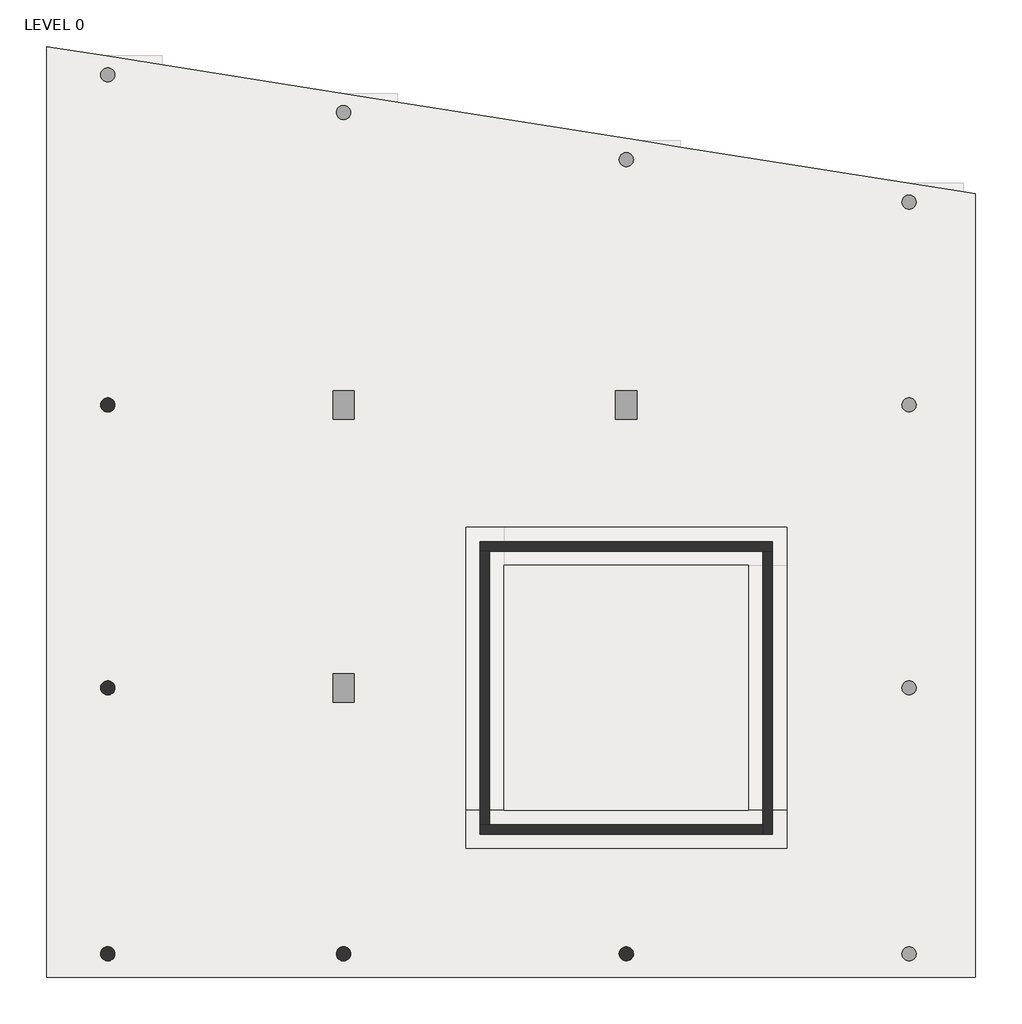
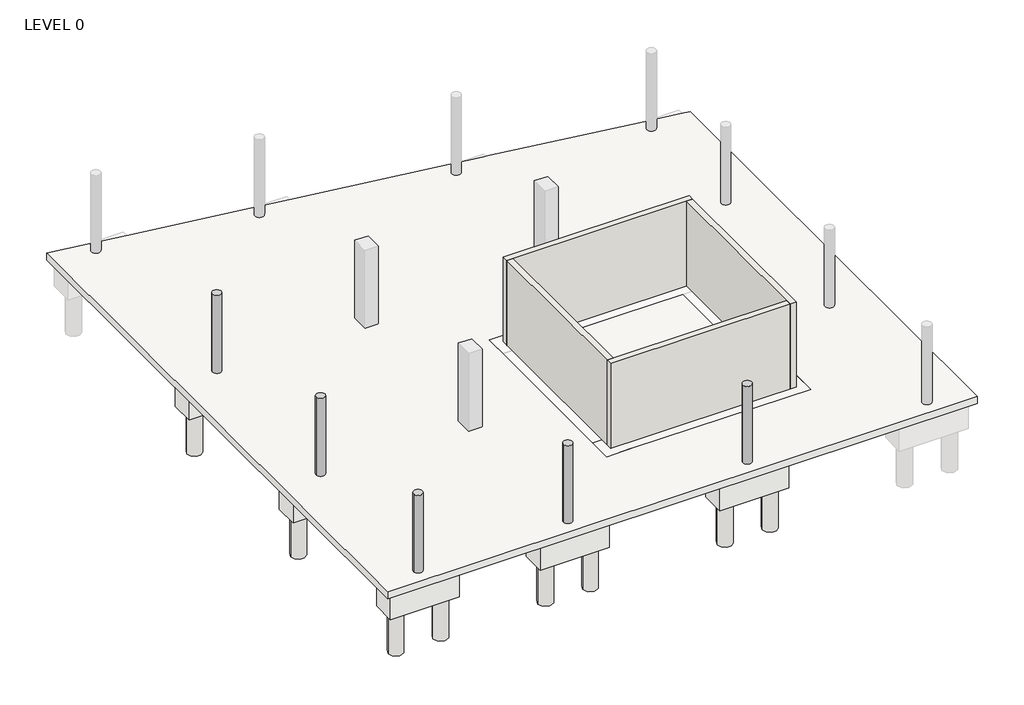
# One storey, part 1 of 3: 14 slabs, 5 columns, 4 walls, 1 footing.
"""IFC4 building model written with IfcOpenShell, lengths in millimetres."""

from ifc_helpers import new_model, si_unit, point, frame, frame_2d, origin, origin_with_axes, place, context, project, spatial, polyline, circle_curve, trimmed, segment, composite_curve, outline, extrude, faceted_brep, element, save
from ifc_brep_helpers import plane_surface, cylinder_surface, revolved_surface, advanced_brep

model = new_model("IFC4")

# Units and contexts
model_context = context("Model", 3, world=origin())
ifc_project = project(units=[si_unit("LENGTHUNIT", "METRE", prefix="MILLI")], contexts=[model_context])

# Site, building, storey
site = spatial("IfcSite", under=ifc_project)
building = spatial("IfcBuilding", under=site)
storey = spatial("IfcBuildingStorey", under=building, Name="LEVEL 0", Elevation=0.0)

# Columns
placement = place(None, origin())
element("IfcColumn", 1, ObjectType="BHm_StructuralColumns_ConcreteRound : 300 Ø RC COL", at=placement, inside=storey, context=model_context, shape_type="SweptSolid", body=[
    extrude(outline(composite_curve([segment(trimmed(circle_curve(frame_2d((-11075.1680269, 3000.0)), 150.0), [point((-11225.1680269, 3000.0))], [point((-10925.1680269, 3000.0))], False, "CARTESIAN"), True, "CONTINUOUS"), segment(trimmed(circle_curve(frame_2d((-11075.1680269, 3000.0)), 150.0), [point((-10925.1680269, 3000.0))], [point((-11225.1680269, 3000.0))], False, "CARTESIAN"), True, "CONTINUOUS")], self_intersect=False)), origin_with_axes(), (0.0, 0.0, 1.0), 2750.0),
])
element("IfcColumn", 2, ObjectType="BHm_StructuralColumns_ConcreteRound : 300 Ø RC COL", at=placement, inside=storey, context=model_context, shape_type="SweptSolid", body=[
    extrude(outline(composite_curve([segment(trimmed(circle_curve(frame_2d((-5075.1680269, 3000.0)), 150.0), [point((-5225.1680269, 3000.0))], [point((-4925.1680269, 3000.0))], False, "CARTESIAN"), True, "CONTINUOUS"), segment(trimmed(circle_curve(frame_2d((-5075.1680269, 3000.0)), 150.0), [point((-4925.1680269, 3000.0))], [point((-5225.1680269, 3000.0))], False, "CARTESIAN"), True, "CONTINUOUS")], self_intersect=False)), origin_with_axes(), (0.0, 0.0, 1.0), 2750.0),
])
element("IfcColumn", 3, ObjectType="BHm_StructuralColumns_ConcreteRound : 300 Ø RC COL", at=placement, inside=storey, context=model_context, shape_type="SweptSolid", body=[
    extrude(outline(composite_curve([segment(trimmed(circle_curve(frame_2d((-16075.1680269, 14640.7845261)), 150.0), [point((-16225.1680269, 14640.7845261))], [point((-15925.1680269, 14640.7845261))], False, "CARTESIAN"), True, "CONTINUOUS"), segment(trimmed(circle_curve(frame_2d((-16075.1680269, 14640.7845261)), 150.0), [point((-15925.1680269, 14640.7845261))], [point((-16225.1680269, 14640.7845261))], False, "CARTESIAN"), True, "CONTINUOUS")], self_intersect=False)), origin_with_axes(), (0.0, 0.0, 1.0), 2750.0),
])
element("IfcColumn", 4, ObjectType="BHm_StructuralColumns_ConcreteRound : 300 Ø RC COL", at=placement, inside=storey, context=model_context, shape_type="SweptSolid", body=[
    extrude(outline(composite_curve([segment(trimmed(circle_curve(frame_2d((-16075.1680269, 8640.7845261)), 150.0), [point((-16225.1680269, 8640.7845261))], [point((-15925.1680269, 8640.7845261))], False, "CARTESIAN"), True, "CONTINUOUS"), segment(trimmed(circle_curve(frame_2d((-16075.1680269, 8640.7845261)), 150.0), [point((-15925.1680269, 8640.7845261))], [point((-16225.1680269, 8640.7845261))], False, "CARTESIAN"), True, "CONTINUOUS")], self_intersect=False)), origin_with_axes(), (0.0, 0.0, 1.0), 2750.0),
])
element("IfcColumn", 5, ObjectType="BHm_StructuralColumns_ConcreteRound : 300 Ø RC COL", at=placement, inside=storey, context=model_context, shape_type="SweptSolid", body=[
    extrude(outline(composite_curve([segment(trimmed(circle_curve(frame_2d((-16075.1680269, 3000.0)), 150.0), [point((-16225.1680269, 3000.0))], [point((-15925.1680269, 3000.0))], False, "CARTESIAN"), True, "CONTINUOUS"), segment(trimmed(circle_curve(frame_2d((-16075.1680269, 3000.0)), 150.0), [point((-15925.1680269, 3000.0))], [point((-16225.1680269, 3000.0))], False, "CARTESIAN"), True, "CONTINUOUS")], self_intersect=False)), origin_with_axes(), (0.0, 0.0, 1.0), 2750.0),
])

# Footing
element("IfcFooting", 6, ObjectType="Wall Foundation", at=placement, inside=storey, context=model_context, shape_type="Brep", body=[
    faceted_brep([(-1670.3680269, 6045.5845261, 0.0), (-2479.9680269, 6045.5845261, 0.0), (-7670.3680269, 6045.5845261, 0.0), (-8479.9680269, 6045.5845261, 0.0), (-8479.9680269, 5235.9845261, 0.0), (-1670.3680269, 5235.9845261, 0.0), (-1670.3680269, 5235.9845261, -500.0), (-1670.3680269, 5235.9845261, -250.0), (-8479.9680269, 5235.9845261, -250.0), (-8479.9680269, 5235.9845261, -500.0), (-1670.3680269, 6045.5845261, -500.0), (-8479.9680269, 6045.5845261, -500.0)], [[[0, 1, 2, 3, 4, 5]], [[6, 7, 5, 4, 8, 9]], [[10, 6, 9, 11]], [[0, 10, 11, 3, 2, 1]], [[0, 5, 7, 6, 10]], [[4, 3, 11, 9, 8]]]),
])

# Slabs
element("IfcSlab", 7, ObjectType="BHm_StructuralFoundations_RC-2PileCap : 500Ø R.C. 2-PILE CAP", at=placement, inside=storey, context=model_context, shape_type="AdvancedBrep", body=[
    advanced_brep(
    [(-9925.1680269, 3400.0, -1100.0), (-9925.1680269, 2600.0, -1100.0), (-12225.1680269, 2600.0, -1100.0), (-12225.1680269, 3400.0, -1100.0), (-12075.1680269, 3000.0, -1100.0), (-11575.1680269, 3000.0, -1100.0), (-10575.1680269, 3000.0, -1100.0), (-10075.1680269, 3000.0, -1100.0), (-12225.1680269, 3400.0, -250.0), (-9925.1680269, 3400.0, -250.0), (-12225.1680269, 2600.0, -250.0), (-9925.1680269, 2600.0, -250.0), (-10575.1680269, 3000.0, -1025.0), (-10075.1680269, 3000.0, -1025.0), (-12075.1680269, 3000.0, -1025.0), (-11575.1680269, 3000.0, -1025.0)],
    [
        (0, 1),
        (1, 2),
        (2, 3),
        (3, 0),
        (4, 5, circle_curve(frame((-11825.1680269, 3000.0, -1100.0), z_axis=(0.0, 0.0, 1.0), x_axis=(1.0, 0.0, 0.0)), 250.0)),
        (5, 4, circle_curve(frame((-11825.1680269, 3000.0, -1100.0), z_axis=(0.0, 0.0, 1.0), x_axis=(1.0, 0.0, 0.0)), 250.0)),
        (6, 7, circle_curve(frame((-10325.1680269, 3000.0, -1100.0), z_axis=(0.0, 0.0, 1.0), x_axis=(1.0, 0.0, 0.0)), 250.0)),
        (7, 6, circle_curve(frame((-10325.1680269, 3000.0, -1100.0), z_axis=(0.0, 0.0, 1.0), x_axis=(1.0, 0.0, 0.0)), 250.0)),
        (3, 8),
        (8, 9),
        (9, 0),
        (2, 10),
        (10, 8),
        (1, 11),
        (11, 10),
        (9, 11),
        (12, 13, circle_curve(frame((-10325.1680269, 3000.0, -1025.0), z_axis=(0.0, 0.0, -1.0), x_axis=(1.0, 0.0, 0.0)), 250.0)),
        (13, 12, circle_curve(frame((-10325.1680269, 3000.0, -1025.0), z_axis=(0.0, 0.0, -1.0), x_axis=(1.0, 0.0, 0.0)), 250.0)),
        (4, 14),
        (14, 15, circle_curve(frame((-11825.1680269, 3000.0, -1025.0), z_axis=(0.0, 0.0, 1.0), x_axis=(1.0, 0.0, 0.0)), 250.0)),
        (15, 5),
        (15, 14, circle_curve(frame((-11825.1680269, 3000.0, -1025.0), z_axis=(0.0, 0.0, 1.0), x_axis=(1.0, 0.0, 0.0)), 250.0)),
        (6, 12),
        (13, 7),
    ],
    [
        plane_surface(frame((-12225.1680269, 3400.0, -1100.0), z_axis=(0.0, 0.0, -1.0), x_axis=(1.0, 0.0, 0.0))),
        plane_surface(frame((-9925.1680269, 3400.0, 0.0), z_axis=(0.0, 1.0, 0.0), x_axis=(0.0, 0.0, -1.0))),
        plane_surface(frame((-12225.1680269, 3400.0, 0.0), z_axis=(-1.0, 0.0, 0.0), x_axis=(0.0, 0.0, -1.0))),
        plane_surface(frame((-12225.1680269, 2600.0, 0.0), z_axis=(0.0, -1.0, 0.0), x_axis=(0.0, 0.0, -1.0))),
        plane_surface(frame((-9925.1680269, 2600.0, 0.0), z_axis=(1.0, 0.0, 0.0), x_axis=(0.0, 0.0, -1.0))),
        plane_surface(frame((-11575.1680269, 3000.0, -1025.0), z_axis=(0.0, 0.0, -1.0), x_axis=(0.0, 1.0, 0.0))),
        revolved_surface(polyline([(-11575.1680269, 3000.0, -1025.0), (-11575.1680269, 3000.0, -1100.0)]), (-11825.1680269, 3000.0, -1100.0), (0.0, 0.0, 1.0)),
        revolved_surface(polyline([(-10075.1680269, 3000.0, -1025.0), (-10075.1680269, 3000.0, -1100.0)]), (-10325.1680269, 3000.0, 0.0), (0.0, 0.0, 1.0)),
        plane_surface(frame((2324.8319731, 15140.7845261, -250.0), z_axis=(0.0, 0.0, 1.0), x_axis=(0.0, -1.0, 0.0))),
    ],
    [
        (0, [[1, 2, 3, 4], [5, 6], [7, 8]]),
        (1, [[-4, 9, 10, 11]]),
        (2, [[-3, 12, 13, -9]]),
        (3, [[-2, 14, 15, -12]]),
        (4, [[-1, -11, 16, -14]]),
        (5, [[17, 18]]),
        (6, [[-5, 19, 20, 21]]),
        (6, [[-6, -21, 22, -19]]),
        (7, [[-7, 23, -18, 24]]),
        (7, [[-8, -24, -17, -23]]),
        (8, [[-10, -13, -15, -16]]),
        (5, [[-22, -20]]),
    ],
),
])
element("IfcSlab", 8, ObjectType="BHm_StructuralFoundations_RC-Pile : 500Ø R.C. PILE", at=placement, inside=storey, context=model_context, shape_type="AdvancedBrep", body=[
    advanced_brep(
    [(-12075.1680269, 3000.0, -1025.0), (-11575.1680269, 3000.0, -1025.0), (-12075.1680269, 3000.0, -2600.0), (-11575.1680269, 3000.0, -2600.0), (-12075.1680269, 3000.0, -1100.0), (-11575.1680269, 3000.0, -1100.0)],
    [
        (0, 1, circle_curve(frame((-11825.1680269, 3000.0, -1025.0), z_axis=(0.0, 0.0, 1.0), x_axis=(1.0, 0.0, 0.0)), 250.0)),
        (1, 0, circle_curve(frame((-11825.1680269, 3000.0, -1025.0), z_axis=(0.0, 0.0, 1.0), x_axis=(1.0, 0.0, 0.0)), 250.0)),
        (2, 3, circle_curve(frame((-11825.1680269, 3000.0, -2600.0), z_axis=(0.0, 0.0, -1.0), x_axis=(1.0, 0.0, 0.0)), 250.0)),
        (3, 2, circle_curve(frame((-11825.1680269, 3000.0, -2600.0), z_axis=(0.0, 0.0, -1.0), x_axis=(1.0, 0.0, 0.0)), 250.0)),
        (0, 4),
        (4, 2),
        (3, 5),
        (5, 1),
    ],
    [
        plane_surface(frame((-11575.1680269, 3000.0, -1025.0), z_axis=(0.0, 0.0, 1.0), x_axis=(0.0, 1.0, 0.0))),
        plane_surface(frame((-11575.1680269, 3000.0, -2600.0), z_axis=(0.0, 0.0, -1.0), x_axis=(0.0, -1.0, 0.0))),
        cylinder_surface(frame((-11825.1680269, 3000.0, -2600.0), z_axis=(0.0, 0.0, 1.0), x_axis=(1.0, 0.0, 0.0)), 250.0),
    ],
    [
        (0, [[1, 2]]),
        (1, [[3, 4]]),
        (2, [[-1, 5, 6, -4, 7, 8]]),
        (2, [[-2, -8, -7, -3, -6, -5]]),
    ],
),
])
element("IfcSlab", 9, ObjectType="BHm_StructuralFoundations_RC-Pile : 500Ø R.C. PILE", at=placement, inside=storey, context=model_context, shape_type="AdvancedBrep", body=[
    advanced_brep(
    [(-10575.1680269, 3000.0, -1025.0), (-10075.1680269, 3000.0, -1025.0), (-10575.1680269, 3000.0, -2600.0), (-10075.1680269, 3000.0, -2600.0), (-10575.1680269, 3000.0, -1100.0), (-10075.1680269, 3000.0, -1100.0)],
    [
        (0, 1, circle_curve(frame((-10325.1680269, 3000.0, -1025.0), z_axis=(0.0, 0.0, 1.0), x_axis=(1.0, 0.0, 0.0)), 250.0)),
        (1, 0, circle_curve(frame((-10325.1680269, 3000.0, -1025.0), z_axis=(0.0, 0.0, 1.0), x_axis=(1.0, 0.0, 0.0)), 250.0)),
        (2, 3, circle_curve(frame((-10325.1680269, 3000.0, -2600.0), z_axis=(0.0, 0.0, -1.0), x_axis=(1.0, 0.0, 0.0)), 250.0)),
        (3, 2, circle_curve(frame((-10325.1680269, 3000.0, -2600.0), z_axis=(0.0, 0.0, -1.0), x_axis=(1.0, 0.0, 0.0)), 250.0)),
        (0, 4),
        (4, 2),
        (3, 5),
        (5, 1),
    ],
    [
        plane_surface(frame((-10075.1680269, 3000.0, -1025.0), z_axis=(0.0, 0.0, 1.0), x_axis=(0.0, 1.0, 0.0))),
        plane_surface(frame((-10075.1680269, 3000.0, -2600.0), z_axis=(0.0, 0.0, -1.0), x_axis=(0.0, -1.0, 0.0))),
        cylinder_surface(frame((-10325.1680269, 3000.0, -2600.0), z_axis=(0.0, 0.0, 1.0), x_axis=(1.0, 0.0, 0.0)), 250.0),
    ],
    [
        (0, [[1, 2]]),
        (1, [[3, 4]]),
        (2, [[-1, 5, 6, -4, 7, 8]]),
        (2, [[-2, -8, -7, -3, -6, -5]]),
    ],
),
])
element("IfcSlab", 10, ObjectType="BHm_StructuralFoundations_RC-2PileCap : 500Ø R.C. 2-PILE CAP", at=placement, inside=storey, context=model_context, shape_type="AdvancedBrep", body=[
    advanced_brep(
    [(-3925.1680269, 3400.0, -1100.0), (-3925.1680269, 2600.0, -1100.0), (-6225.1680269, 2600.0, -1100.0), (-6225.1680269, 3400.0, -1100.0), (-6075.1680269, 3000.0, -1100.0), (-5575.1680269, 3000.0, -1100.0), (-4575.1680269, 3000.0, -1100.0), (-4075.1680269, 3000.0, -1100.0), (-6225.1680269, 3400.0, -250.0), (-3925.1680269, 3400.0, -250.0), (-6225.1680269, 2600.0, -250.0), (-3925.1680269, 2600.0, -250.0), (-4575.1680269, 3000.0, -1025.0), (-4075.1680269, 3000.0, -1025.0), (-6075.1680269, 3000.0, -1025.0), (-5575.1680269, 3000.0, -1025.0)],
    [
        (0, 1),
        (1, 2),
        (2, 3),
        (3, 0),
        (4, 5, circle_curve(frame((-5825.1680269, 3000.0, -1100.0), z_axis=(0.0, 0.0, 1.0), x_axis=(1.0, 0.0, 0.0)), 250.0)),
        (5, 4, circle_curve(frame((-5825.1680269, 3000.0, -1100.0), z_axis=(0.0, 0.0, 1.0), x_axis=(1.0, 0.0, 0.0)), 250.0)),
        (6, 7, circle_curve(frame((-4325.1680269, 3000.0, -1100.0), z_axis=(0.0, 0.0, 1.0), x_axis=(1.0, 0.0, 0.0)), 250.0)),
        (7, 6, circle_curve(frame((-4325.1680269, 3000.0, -1100.0), z_axis=(0.0, 0.0, 1.0), x_axis=(1.0, 0.0, 0.0)), 250.0)),
        (3, 8),
        (8, 9),
        (9, 0),
        (2, 10),
        (10, 8),
        (1, 11),
        (11, 10),
        (9, 11),
        (12, 13, circle_curve(frame((-4325.1680269, 3000.0, -1025.0), z_axis=(0.0, 0.0, -1.0), x_axis=(1.0, 0.0, 0.0)), 250.0)),
        (13, 12, circle_curve(frame((-4325.1680269, 3000.0, -1025.0), z_axis=(0.0, 0.0, -1.0), x_axis=(1.0, 0.0, 0.0)), 250.0)),
        (4, 14),
        (14, 15, circle_curve(frame((-5825.1680269, 3000.0, -1025.0), z_axis=(0.0, 0.0, 1.0), x_axis=(1.0, 0.0, 0.0)), 250.0)),
        (15, 5),
        (15, 14, circle_curve(frame((-5825.1680269, 3000.0, -1025.0), z_axis=(0.0, 0.0, 1.0), x_axis=(1.0, 0.0, 0.0)), 250.0)),
        (6, 12),
        (13, 7),
    ],
    [
        plane_surface(frame((-6225.1680269, 3400.0, -1100.0), z_axis=(0.0, 0.0, -1.0), x_axis=(1.0, 0.0, 0.0))),
        plane_surface(frame((-3925.1680269, 3400.0, 0.0), z_axis=(0.0, 1.0, 0.0), x_axis=(0.0, 0.0, -1.0))),
        plane_surface(frame((-6225.1680269, 3400.0, 0.0), z_axis=(-1.0, 0.0, 0.0), x_axis=(0.0, 0.0, -1.0))),
        plane_surface(frame((-6225.1680269, 2600.0, 0.0), z_axis=(0.0, -1.0, 0.0), x_axis=(0.0, 0.0, -1.0))),
        plane_surface(frame((-3925.1680269, 2600.0, 0.0), z_axis=(1.0, 0.0, 0.0), x_axis=(0.0, 0.0, -1.0))),
        plane_surface(frame((-5575.1680269, 3000.0, -1025.0), z_axis=(0.0, 0.0, -1.0), x_axis=(0.0, 1.0, 0.0))),
        revolved_surface(polyline([(-5575.1680269, 3000.0, -1025.0), (-5575.1680269, 3000.0, -1100.0)]), (-5825.1680269, 3000.0, -1100.0), (0.0, 0.0, 1.0)),
        revolved_surface(polyline([(-4075.1680269, 3000.0, -1025.0), (-4075.1680269, 3000.0, -1100.0)]), (-4325.1680269, 3000.0, 0.0), (0.0, 0.0, 1.0)),
        plane_surface(frame((2324.8319731, 15140.7845261, -250.0), z_axis=(0.0, 0.0, 1.0), x_axis=(0.0, -1.0, 0.0))),
    ],
    [
        (0, [[1, 2, 3, 4], [5, 6], [7, 8]]),
        (1, [[-4, 9, 10, 11]]),
        (2, [[-3, 12, 13, -9]]),
        (3, [[-2, 14, 15, -12]]),
        (4, [[-1, -11, 16, -14]]),
        (5, [[17, 18]]),
        (6, [[-5, 19, 20, 21]]),
        (6, [[-6, -21, 22, -19]]),
        (7, [[-7, 23, -18, 24]]),
        (7, [[-8, -24, -17, -23]]),
        (8, [[-10, -13, -15, -16]]),
        (5, [[-22, -20]]),
    ],
),
])
element("IfcSlab", 11, ObjectType="BHm_StructuralFoundations_RC-Pile : 500Ø R.C. PILE", at=placement, inside=storey, context=model_context, shape_type="AdvancedBrep", body=[
    advanced_brep(
    [(-6075.1680269, 3000.0, -1025.0), (-5575.1680269, 3000.0, -1025.0), (-6075.1680269, 3000.0, -2600.0), (-5575.1680269, 3000.0, -2600.0), (-6075.1680269, 3000.0, -1100.0), (-5575.1680269, 3000.0, -1100.0)],
    [
        (0, 1, circle_curve(frame((-5825.1680269, 3000.0, -1025.0), z_axis=(0.0, 0.0, 1.0), x_axis=(1.0, 0.0, 0.0)), 250.0)),
        (1, 0, circle_curve(frame((-5825.1680269, 3000.0, -1025.0), z_axis=(0.0, 0.0, 1.0), x_axis=(1.0, 0.0, 0.0)), 250.0)),
        (2, 3, circle_curve(frame((-5825.1680269, 3000.0, -2600.0), z_axis=(0.0, 0.0, -1.0), x_axis=(1.0, 0.0, 0.0)), 250.0)),
        (3, 2, circle_curve(frame((-5825.1680269, 3000.0, -2600.0), z_axis=(0.0, 0.0, -1.0), x_axis=(1.0, 0.0, 0.0)), 250.0)),
        (0, 4),
        (4, 2),
        (3, 5),
        (5, 1),
    ],
    [
        plane_surface(frame((-5575.1680269, 3000.0, -1025.0), z_axis=(0.0, 0.0, 1.0), x_axis=(0.0, 1.0, 0.0))),
        plane_surface(frame((-5575.1680269, 3000.0, -2600.0), z_axis=(0.0, 0.0, -1.0), x_axis=(0.0, -1.0, 0.0))),
        cylinder_surface(frame((-5825.1680269, 3000.0, -2600.0), z_axis=(0.0, 0.0, 1.0), x_axis=(1.0, 0.0, 0.0)), 250.0),
    ],
    [
        (0, [[1, 2]]),
        (1, [[3, 4]]),
        (2, [[-1, 5, 6, -4, 7, 8]]),
        (2, [[-2, -8, -7, -3, -6, -5]]),
    ],
),
])
element("IfcSlab", 12, ObjectType="BHm_StructuralFoundations_RC-Pile : 500Ø R.C. PILE", at=placement, inside=storey, context=model_context, shape_type="AdvancedBrep", body=[
    advanced_brep(
    [(-4575.1680269, 3000.0, -1025.0), (-4075.1680269, 3000.0, -1025.0), (-4575.1680269, 3000.0, -2600.0), (-4075.1680269, 3000.0, -2600.0), (-4575.1680269, 3000.0, -1100.0), (-4075.1680269, 3000.0, -1100.0)],
    [
        (0, 1, circle_curve(frame((-4325.1680269, 3000.0, -1025.0), z_axis=(0.0, 0.0, 1.0), x_axis=(1.0, 0.0, 0.0)), 250.0)),
        (1, 0, circle_curve(frame((-4325.1680269, 3000.0, -1025.0), z_axis=(0.0, 0.0, 1.0), x_axis=(1.0, 0.0, 0.0)), 250.0)),
        (2, 3, circle_curve(frame((-4325.1680269, 3000.0, -2600.0), z_axis=(0.0, 0.0, -1.0), x_axis=(1.0, 0.0, 0.0)), 250.0)),
        (3, 2, circle_curve(frame((-4325.1680269, 3000.0, -2600.0), z_axis=(0.0, 0.0, -1.0), x_axis=(1.0, 0.0, 0.0)), 250.0)),
        (0, 4),
        (4, 2),
        (3, 5),
        (5, 1),
    ],
    [
        plane_surface(frame((-4075.1680269, 3000.0, -1025.0), z_axis=(0.0, 0.0, 1.0), x_axis=(0.0, 1.0, 0.0))),
        plane_surface(frame((-4075.1680269, 3000.0, -2600.0), z_axis=(0.0, 0.0, -1.0), x_axis=(0.0, -1.0, 0.0))),
        cylinder_surface(frame((-4325.1680269, 3000.0, -2600.0), z_axis=(0.0, 0.0, 1.0), x_axis=(1.0, 0.0, 0.0)), 250.0),
    ],
    [
        (0, [[1, 2]]),
        (1, [[3, 4]]),
        (2, [[-1, 5, 6, -4, 7, 8]]),
        (2, [[-2, -8, -7, -3, -6, -5]]),
    ],
),
])
element("IfcSlab", 13, ObjectType="BHm_StructuralFoundations_RC-2PileCap : 500Ø R.C. 2-PILE CAP", at=placement, inside=storey, context=model_context, shape_type="AdvancedBrep", body=[
    advanced_brep(
    [(-14925.1680269, 15040.7845261, -1100.0), (-14925.1680269, 14240.7845261, -1100.0), (-17225.1680269, 14240.7845261, -1100.0), (-17225.1680269, 15040.7845261, -1100.0), (-17075.1680269, 14640.7845261, -1100.0), (-16575.1680269, 14640.7845261, -1100.0), (-15575.1680269, 14640.7845261, -1100.0), (-15075.1680269, 14640.7845261, -1100.0), (-17225.1680269, 15040.7845261, -250.0), (-14925.1680269, 15040.7845261, -250.0), (-17225.1680269, 14240.7845261, -250.0), (-14925.1680269, 14240.7845261, -250.0), (-15575.1680269, 14640.7845261, -1025.0), (-15075.1680269, 14640.7845261, -1025.0), (-17075.1680269, 14640.7845261, -1025.0), (-16575.1680269, 14640.7845261, -1025.0)],
    [
        (0, 1),
        (1, 2),
        (2, 3),
        (3, 0),
        (4, 5, circle_curve(frame((-16825.1680269, 14640.7845261, -1100.0), z_axis=(0.0, 0.0, 1.0), x_axis=(1.0, 0.0, 0.0)), 250.0)),
        (5, 4, circle_curve(frame((-16825.1680269, 14640.7845261, -1100.0), z_axis=(0.0, 0.0, 1.0), x_axis=(1.0, 0.0, 0.0)), 250.0)),
        (6, 7, circle_curve(frame((-15325.1680269, 14640.7845261, -1100.0), z_axis=(0.0, 0.0, 1.0), x_axis=(1.0, 0.0, 0.0)), 250.0)),
        (7, 6, circle_curve(frame((-15325.1680269, 14640.7845261, -1100.0), z_axis=(0.0, 0.0, 1.0), x_axis=(1.0, 0.0, 0.0)), 250.0)),
        (3, 8),
        (8, 9),
        (9, 0),
        (2, 10),
        (10, 8),
        (1, 11),
        (11, 10),
        (9, 11),
        (12, 13, circle_curve(frame((-15325.1680269, 14640.7845261, -1025.0), z_axis=(0.0, 0.0, -1.0), x_axis=(1.0, 0.0, 0.0)), 250.0)),
        (13, 12, circle_curve(frame((-15325.1680269, 14640.7845261, -1025.0), z_axis=(0.0, 0.0, -1.0), x_axis=(1.0, 0.0, 0.0)), 250.0)),
        (4, 14),
        (14, 15, circle_curve(frame((-16825.1680269, 14640.7845261, -1025.0), z_axis=(0.0, 0.0, 1.0), x_axis=(1.0, 0.0, 0.0)), 250.0)),
        (15, 5),
        (15, 14, circle_curve(frame((-16825.1680269, 14640.7845261, -1025.0), z_axis=(0.0, 0.0, 1.0), x_axis=(1.0, 0.0, 0.0)), 250.0)),
        (6, 12),
        (13, 7),
    ],
    [
        plane_surface(frame((-17225.1680269, 15040.7845261, -1100.0), z_axis=(0.0, 0.0, -1.0), x_axis=(1.0, 0.0, 0.0))),
        plane_surface(frame((-14925.1680269, 15040.7845261, 0.0), z_axis=(0.0, 1.0, 0.0), x_axis=(0.0, 0.0, -1.0))),
        plane_surface(frame((-17225.1680269, 15040.7845261, 0.0), z_axis=(-1.0, 0.0, 0.0), x_axis=(0.0, 0.0, -1.0))),
        plane_surface(frame((-17225.1680269, 14240.7845261, 0.0), z_axis=(0.0, -1.0, 0.0), x_axis=(0.0, 0.0, -1.0))),
        plane_surface(frame((-14925.1680269, 14240.7845261, 0.0), z_axis=(1.0, 0.0, 0.0), x_axis=(0.0, 0.0, -1.0))),
        plane_surface(frame((-16575.1680269, 14640.7845261, -1025.0), z_axis=(0.0, 0.0, -1.0), x_axis=(0.0, 1.0, 0.0))),
        revolved_surface(polyline([(-16575.1680269, 14640.7845261, -1025.0), (-16575.1680269, 14640.7845261, -1100.0)]), (-16825.1680269, 14640.7845261, -1100.0), (0.0, 0.0, 1.0)),
        revolved_surface(polyline([(-15075.1680269, 14640.7845261, -1025.0), (-15075.1680269, 14640.7845261, -1100.0)]), (-15325.1680269, 14640.7845261, 0.0), (0.0, 0.0, 1.0)),
        plane_surface(frame((2324.8319731, 15140.7845261, -250.0), z_axis=(0.0, 0.0, 1.0), x_axis=(0.0, -1.0, 0.0))),
    ],
    [
        (0, [[1, 2, 3, 4], [5, 6], [7, 8]]),
        (1, [[-4, 9, 10, 11]]),
        (2, [[-3, 12, 13, -9]]),
        (3, [[-2, 14, 15, -12]]),
        (4, [[-1, -11, 16, -14]]),
        (5, [[17, 18]]),
        (6, [[-5, 19, 20, 21]]),
        (6, [[-6, -21, 22, -19]]),
        (7, [[-7, 23, -18, 24]]),
        (7, [[-8, -24, -17, -23]]),
        (8, [[-10, -13, -15, -16]]),
        (5, [[-22, -20]]),
    ],
),
])
element("IfcSlab", 14, ObjectType="BHm_StructuralFoundations_RC-Pile : 500Ø R.C. PILE", at=placement, inside=storey, context=model_context, shape_type="AdvancedBrep", body=[
    advanced_brep(
    [(-17075.1680269, 14640.7845261, -1025.0), (-16575.1680269, 14640.7845261, -1025.0), (-17075.1680269, 14640.7845261, -2600.0), (-16575.1680269, 14640.7845261, -2600.0), (-17075.1680269, 14640.7845261, -1100.0), (-16575.1680269, 14640.7845261, -1100.0)],
    [
        (0, 1, circle_curve(frame((-16825.1680269, 14640.7845261, -1025.0), z_axis=(0.0, 0.0, 1.0), x_axis=(1.0, 0.0, 0.0)), 250.0)),
        (1, 0, circle_curve(frame((-16825.1680269, 14640.7845261, -1025.0), z_axis=(0.0, 0.0, 1.0), x_axis=(1.0, 0.0, 0.0)), 250.0)),
        (2, 3, circle_curve(frame((-16825.1680269, 14640.7845261, -2600.0), z_axis=(0.0, 0.0, -1.0), x_axis=(1.0, 0.0, 0.0)), 250.0)),
        (3, 2, circle_curve(frame((-16825.1680269, 14640.7845261, -2600.0), z_axis=(0.0, 0.0, -1.0), x_axis=(1.0, 0.0, 0.0)), 250.0)),
        (0, 4),
        (4, 2),
        (3, 5),
        (5, 1),
    ],
    [
        plane_surface(frame((-16575.1680269, 14640.7845261, -1025.0), z_axis=(0.0, 0.0, 1.0), x_axis=(0.0, 1.0, 0.0))),
        plane_surface(frame((-16575.1680269, 14640.7845261, -2600.0), z_axis=(0.0, 0.0, -1.0), x_axis=(0.0, -1.0, 0.0))),
        cylinder_surface(frame((-16825.1680269, 14640.7845261, -2600.0), z_axis=(0.0, 0.0, 1.0), x_axis=(1.0, 0.0, 0.0)), 250.0),
    ],
    [
        (0, [[1, 2]]),
        (1, [[3, 4]]),
        (2, [[-1, 5, 6, -4, 7, 8]]),
        (2, [[-2, -8, -7, -3, -6, -5]]),
    ],
),
])
element("IfcSlab", 15, ObjectType="BHm_StructuralFoundations_RC-2PileCap : 500Ø R.C. 2-PILE CAP", at=placement, inside=storey, context=model_context, shape_type="AdvancedBrep", body=[
    advanced_brep(
    [(-14925.1680269, 9040.7845261, -1100.0), (-14925.1680269, 8240.7845261, -1100.0), (-17225.1680269, 8240.7845261, -1100.0), (-17225.1680269, 9040.7845261, -1100.0), (-17075.1680269, 8640.7845261, -1100.0), (-16575.1680269, 8640.7845261, -1100.0), (-15575.1680269, 8640.7845261, -1100.0), (-15075.1680269, 8640.7845261, -1100.0), (-17225.1680269, 9040.7845261, -250.0), (-14925.1680269, 9040.7845261, -250.0), (-17225.1680269, 8240.7845261, -250.0), (-14925.1680269, 8240.7845261, -250.0), (-15575.1680269, 8640.7845261, -1025.0), (-15075.1680269, 8640.7845261, -1025.0), (-17075.1680269, 8640.7845261, -1025.0), (-16575.1680269, 8640.7845261, -1025.0)],
    [
        (0, 1),
        (1, 2),
        (2, 3),
        (3, 0),
        (4, 5, circle_curve(frame((-16825.1680269, 8640.7845261, -1100.0), z_axis=(0.0, 0.0, 1.0), x_axis=(1.0, 0.0, 0.0)), 250.0)),
        (5, 4, circle_curve(frame((-16825.1680269, 8640.7845261, -1100.0), z_axis=(0.0, 0.0, 1.0), x_axis=(1.0, 0.0, 0.0)), 250.0)),
        (6, 7, circle_curve(frame((-15325.1680269, 8640.7845261, -1100.0), z_axis=(0.0, 0.0, 1.0), x_axis=(1.0, 0.0, 0.0)), 250.0)),
        (7, 6, circle_curve(frame((-15325.1680269, 8640.7845261, -1100.0), z_axis=(0.0, 0.0, 1.0), x_axis=(1.0, 0.0, 0.0)), 250.0)),
        (3, 8),
        (8, 9),
        (9, 0),
        (2, 10),
        (10, 8),
        (1, 11),
        (11, 10),
        (9, 11),
        (12, 13, circle_curve(frame((-15325.1680269, 8640.7845261, -1025.0), z_axis=(0.0, 0.0, -1.0), x_axis=(1.0, 0.0, 0.0)), 250.0)),
        (13, 12, circle_curve(frame((-15325.1680269, 8640.7845261, -1025.0), z_axis=(0.0, 0.0, -1.0), x_axis=(1.0, 0.0, 0.0)), 250.0)),
        (4, 14),
        (14, 15, circle_curve(frame((-16825.1680269, 8640.7845261, -1025.0), z_axis=(0.0, 0.0, 1.0), x_axis=(1.0, 0.0, 0.0)), 250.0)),
        (15, 5),
        (15, 14, circle_curve(frame((-16825.1680269, 8640.7845261, -1025.0), z_axis=(0.0, 0.0, 1.0), x_axis=(1.0, 0.0, 0.0)), 250.0)),
        (6, 12),
        (13, 7),
    ],
    [
        plane_surface(frame((-17225.1680269, 9040.7845261, -1100.0), z_axis=(0.0, 0.0, -1.0), x_axis=(1.0, 0.0, 0.0))),
        plane_surface(frame((-14925.1680269, 9040.7845261, 0.0), z_axis=(0.0, 1.0, 0.0), x_axis=(0.0, 0.0, -1.0))),
        plane_surface(frame((-17225.1680269, 9040.7845261, 0.0), z_axis=(-1.0, 0.0, 0.0), x_axis=(0.0, 0.0, -1.0))),
        plane_surface(frame((-17225.1680269, 8240.7845261, 0.0), z_axis=(0.0, -1.0, 0.0), x_axis=(0.0, 0.0, -1.0))),
        plane_surface(frame((-14925.1680269, 8240.7845261, 0.0), z_axis=(1.0, 0.0, 0.0), x_axis=(0.0, 0.0, -1.0))),
        plane_surface(frame((-16575.1680269, 8640.7845261, -1025.0), z_axis=(0.0, 0.0, -1.0), x_axis=(0.0, 1.0, 0.0))),
        revolved_surface(polyline([(-16575.1680269, 8640.7845261, -1025.0), (-16575.1680269, 8640.7845261, -1100.0)]), (-16825.1680269, 8640.7845261, -1100.0), (0.0, 0.0, 1.0)),
        revolved_surface(polyline([(-15075.1680269, 8640.7845261, -1025.0), (-15075.1680269, 8640.7845261, -1100.0)]), (-15325.1680269, 8640.7845261, 0.0), (0.0, 0.0, 1.0)),
        plane_surface(frame((2324.8319731, 15140.7845261, -250.0), z_axis=(0.0, 0.0, 1.0), x_axis=(0.0, -1.0, 0.0))),
    ],
    [
        (0, [[1, 2, 3, 4], [5, 6], [7, 8]]),
        (1, [[-4, 9, 10, 11]]),
        (2, [[-3, 12, 13, -9]]),
        (3, [[-2, 14, 15, -12]]),
        (4, [[-1, -11, 16, -14]]),
        (5, [[17, 18]]),
        (6, [[-5, 19, 20, 21]]),
        (6, [[-6, -21, 22, -19]]),
        (7, [[-7, 23, -18, 24]]),
        (7, [[-8, -24, -17, -23]]),
        (8, [[-10, -13, -15, -16]]),
        (5, [[-22, -20]]),
    ],
),
])
element("IfcSlab", 16, ObjectType="BHm_StructuralFoundations_RC-Pile : 500Ø R.C. PILE", at=placement, inside=storey, context=model_context, shape_type="AdvancedBrep", body=[
    advanced_brep(
    [(-17075.1680269, 8640.7845261, -1025.0), (-16575.1680269, 8640.7845261, -1025.0), (-17075.1680269, 8640.7845261, -2600.0), (-16575.1680269, 8640.7845261, -2600.0), (-17075.1680269, 8640.7845261, -1100.0), (-16575.1680269, 8640.7845261, -1100.0)],
    [
        (0, 1, circle_curve(frame((-16825.1680269, 8640.7845261, -1025.0), z_axis=(0.0, 0.0, 1.0), x_axis=(1.0, 0.0, 0.0)), 250.0)),
        (1, 0, circle_curve(frame((-16825.1680269, 8640.7845261, -1025.0), z_axis=(0.0, 0.0, 1.0), x_axis=(1.0, 0.0, 0.0)), 250.0)),
        (2, 3, circle_curve(frame((-16825.1680269, 8640.7845261, -2600.0), z_axis=(0.0, 0.0, -1.0), x_axis=(1.0, 0.0, 0.0)), 250.0)),
        (3, 2, circle_curve(frame((-16825.1680269, 8640.7845261, -2600.0), z_axis=(0.0, 0.0, -1.0), x_axis=(1.0, 0.0, 0.0)), 250.0)),
        (0, 4),
        (4, 2),
        (3, 5),
        (5, 1),
    ],
    [
        plane_surface(frame((-16575.1680269, 8640.7845261, -1025.0), z_axis=(0.0, 0.0, 1.0), x_axis=(0.0, 1.0, 0.0))),
        plane_surface(frame((-16575.1680269, 8640.7845261, -2600.0), z_axis=(0.0, 0.0, -1.0), x_axis=(0.0, -1.0, 0.0))),
        cylinder_surface(frame((-16825.1680269, 8640.7845261, -2600.0), z_axis=(0.0, 0.0, 1.0), x_axis=(1.0, 0.0, 0.0)), 250.0),
    ],
    [
        (0, [[1, 2]]),
        (1, [[3, 4]]),
        (2, [[-1, 5, 6, -4, 7, 8]]),
        (2, [[-2, -8, -7, -3, -6, -5]]),
    ],
),
])
element("IfcSlab", 17, ObjectType="BHm_StructuralFoundations_RC-2PileCap : 500Ø R.C. 2-PILE CAP", at=placement, inside=storey, context=model_context, shape_type="AdvancedBrep", body=[
    advanced_brep(
    [(-14925.1680269, 3400.0, -1100.0), (-14925.1680269, 2600.0, -1100.0), (-17225.1680269, 2600.0, -1100.0), (-17225.1680269, 3400.0, -1100.0), (-17075.1680269, 3000.0, -1100.0), (-16575.1680269, 3000.0, -1100.0), (-15575.1680269, 3000.0, -1100.0), (-15075.1680269, 3000.0, -1100.0), (-17225.1680269, 3400.0, -250.0), (-14925.1680269, 3400.0, -250.0), (-17225.1680269, 2600.0, -250.0), (-14925.1680269, 2600.0, -250.0), (-15575.1680269, 3000.0, -1025.0), (-15075.1680269, 3000.0, -1025.0), (-17075.1680269, 3000.0, -1025.0), (-16575.1680269, 3000.0, -1025.0)],
    [
        (0, 1),
        (1, 2),
        (2, 3),
        (3, 0),
        (4, 5, circle_curve(frame((-16825.1680269, 3000.0, -1100.0), z_axis=(0.0, 0.0, 1.0), x_axis=(1.0, 0.0, 0.0)), 250.0)),
        (5, 4, circle_curve(frame((-16825.1680269, 3000.0, -1100.0), z_axis=(0.0, 0.0, 1.0), x_axis=(1.0, 0.0, 0.0)), 250.0)),
        (6, 7, circle_curve(frame((-15325.1680269, 3000.0, -1100.0), z_axis=(0.0, 0.0, 1.0), x_axis=(1.0, 0.0, 0.0)), 250.0)),
        (7, 6, circle_curve(frame((-15325.1680269, 3000.0, -1100.0), z_axis=(0.0, 0.0, 1.0), x_axis=(1.0, 0.0, 0.0)), 250.0)),
        (3, 8),
        (8, 9),
        (9, 0),
        (2, 10),
        (10, 8),
        (1, 11),
        (11, 10),
        (9, 11),
        (12, 13, circle_curve(frame((-15325.1680269, 3000.0, -1025.0), z_axis=(0.0, 0.0, -1.0), x_axis=(1.0, 0.0, 0.0)), 250.0)),
        (13, 12, circle_curve(frame((-15325.1680269, 3000.0, -1025.0), z_axis=(0.0, 0.0, -1.0), x_axis=(1.0, 0.0, 0.0)), 250.0)),
        (4, 14),
        (14, 15, circle_curve(frame((-16825.1680269, 3000.0, -1025.0), z_axis=(0.0, 0.0, 1.0), x_axis=(1.0, 0.0, 0.0)), 250.0)),
        (15, 5),
        (15, 14, circle_curve(frame((-16825.1680269, 3000.0, -1025.0), z_axis=(0.0, 0.0, 1.0), x_axis=(1.0, 0.0, 0.0)), 250.0)),
        (6, 12),
        (13, 7),
    ],
    [
        plane_surface(frame((-17225.1680269, 3400.0, -1100.0), z_axis=(0.0, 0.0, -1.0), x_axis=(1.0, 0.0, 0.0))),
        plane_surface(frame((-14925.1680269, 3400.0, 0.0), z_axis=(0.0, 1.0, 0.0), x_axis=(0.0, 0.0, -1.0))),
        plane_surface(frame((-17225.1680269, 3400.0, 0.0), z_axis=(-1.0, 0.0, 0.0), x_axis=(0.0, 0.0, -1.0))),
        plane_surface(frame((-17225.1680269, 2600.0, 0.0), z_axis=(0.0, -1.0, 0.0), x_axis=(0.0, 0.0, -1.0))),
        plane_surface(frame((-14925.1680269, 2600.0, 0.0), z_axis=(1.0, 0.0, 0.0), x_axis=(0.0, 0.0, -1.0))),
        plane_surface(frame((-16575.1680269, 3000.0, -1025.0), z_axis=(0.0, 0.0, -1.0), x_axis=(0.0, 1.0, 0.0))),
        revolved_surface(polyline([(-16575.1680269, 3000.0, -1025.0), (-16575.1680269, 3000.0, -1100.0)]), (-16825.1680269, 3000.0, -1100.0), (0.0, 0.0, 1.0)),
        revolved_surface(polyline([(-15075.1680269, 3000.0, -1025.0), (-15075.1680269, 3000.0, -1100.0)]), (-15325.1680269, 3000.0, 0.0), (0.0, 0.0, 1.0)),
        plane_surface(frame((2324.8319731, 15140.7845261, -250.0), z_axis=(0.0, 0.0, 1.0), x_axis=(0.0, -1.0, 0.0))),
    ],
    [
        (0, [[1, 2, 3, 4], [5, 6], [7, 8]]),
        (1, [[-4, 9, 10, 11]]),
        (2, [[-3, 12, 13, -9]]),
        (3, [[-2, 14, 15, -12]]),
        (4, [[-1, -11, 16, -14]]),
        (5, [[17, 18]]),
        (6, [[-5, 19, 20, 21]]),
        (6, [[-6, -21, 22, -19]]),
        (7, [[-7, 23, -18, 24]]),
        (7, [[-8, -24, -17, -23]]),
        (8, [[-10, -13, -15, -16]]),
        (5, [[-22, -20]]),
    ],
),
])
element("IfcSlab", 18, ObjectType="BHm_StructuralFoundations_RC-Pile : 500Ø R.C. PILE", at=placement, inside=storey, context=model_context, shape_type="AdvancedBrep", body=[
    advanced_brep(
    [(-17075.1680269, 3000.0, -1025.0), (-16575.1680269, 3000.0, -1025.0), (-17075.1680269, 3000.0, -2600.0), (-16575.1680269, 3000.0, -2600.0), (-17075.1680269, 3000.0, -1100.0), (-16575.1680269, 3000.0, -1100.0)],
    [
        (0, 1, circle_curve(frame((-16825.1680269, 3000.0, -1025.0), z_axis=(0.0, 0.0, 1.0), x_axis=(1.0, 0.0, 0.0)), 250.0)),
        (1, 0, circle_curve(frame((-16825.1680269, 3000.0, -1025.0), z_axis=(0.0, 0.0, 1.0), x_axis=(1.0, 0.0, 0.0)), 250.0)),
        (2, 3, circle_curve(frame((-16825.1680269, 3000.0, -2600.0), z_axis=(0.0, 0.0, -1.0), x_axis=(1.0, 0.0, 0.0)), 250.0)),
        (3, 2, circle_curve(frame((-16825.1680269, 3000.0, -2600.0), z_axis=(0.0, 0.0, -1.0), x_axis=(1.0, 0.0, 0.0)), 250.0)),
        (0, 4),
        (4, 2),
        (3, 5),
        (5, 1),
    ],
    [
        plane_surface(frame((-16575.1680269, 3000.0, -1025.0), z_axis=(0.0, 0.0, 1.0), x_axis=(0.0, 1.0, 0.0))),
        plane_surface(frame((-16575.1680269, 3000.0, -2600.0), z_axis=(0.0, 0.0, -1.0), x_axis=(0.0, -1.0, 0.0))),
        cylinder_surface(frame((-16825.1680269, 3000.0, -2600.0), z_axis=(0.0, 0.0, 1.0), x_axis=(1.0, 0.0, 0.0)), 250.0),
    ],
    [
        (0, [[1, 2]]),
        (1, [[3, 4]]),
        (2, [[-1, 5, 6, -4, 7, 8]]),
        (2, [[-2, -8, -7, -3, -6, -5]]),
    ],
),
])
element("IfcSlab", 19, ObjectType="BHm_StructuralFoundations_RC-Pile : 500Ø R.C. PILE", at=placement, inside=storey, context=model_context, shape_type="AdvancedBrep", body=[
    advanced_brep(
    [(-15575.1680269, 3000.0, -1025.0), (-15075.1680269, 3000.0, -1025.0), (-15575.1680269, 3000.0, -2600.0), (-15075.1680269, 3000.0, -2600.0), (-15575.1680269, 3000.0, -1100.0), (-15075.1680269, 3000.0, -1100.0)],
    [
        (0, 1, circle_curve(frame((-15325.1680269, 3000.0, -1025.0), z_axis=(0.0, 0.0, 1.0), x_axis=(1.0, 0.0, 0.0)), 250.0)),
        (1, 0, circle_curve(frame((-15325.1680269, 3000.0, -1025.0), z_axis=(0.0, 0.0, 1.0), x_axis=(1.0, 0.0, 0.0)), 250.0)),
        (2, 3, circle_curve(frame((-15325.1680269, 3000.0, -2600.0), z_axis=(0.0, 0.0, -1.0), x_axis=(1.0, 0.0, 0.0)), 250.0)),
        (3, 2, circle_curve(frame((-15325.1680269, 3000.0, -2600.0), z_axis=(0.0, 0.0, -1.0), x_axis=(1.0, 0.0, 0.0)), 250.0)),
        (0, 4),
        (4, 2),
        (3, 5),
        (5, 1),
    ],
    [
        plane_surface(frame((-15075.1680269, 3000.0, -1025.0), z_axis=(0.0, 0.0, 1.0), x_axis=(0.0, 1.0, 0.0))),
        plane_surface(frame((-15075.1680269, 3000.0, -2600.0), z_axis=(0.0, 0.0, -1.0), x_axis=(0.0, -1.0, 0.0))),
        cylinder_surface(frame((-15325.1680269, 3000.0, -2600.0), z_axis=(0.0, 0.0, 1.0), x_axis=(1.0, 0.0, 0.0)), 250.0),
    ],
    [
        (0, [[1, 2]]),
        (1, [[3, 4]]),
        (2, [[-1, 5, 6, -4, 7, 8]]),
        (2, [[-2, -8, -7, -3, -6, -5]]),
    ],
),
])
element("IfcSlab", 20, ObjectType="250 THK RC SLAB", at=placement, inside=storey, context=model_context, shape_type="Brep", body=[
    faceted_brep([(2324.8319731, 19120.6110517, -250.0), (2324.8319731, 2500.0, -250.0), (-17375.1680269, 2500.0, -250.0), (-17375.1680269, 22240.7845261, -250.0), (-16112.417724, 22040.7845261, -250.0), (-14925.1680269, 21852.7426473, -250.0), (-11061.4165123, 21240.7845261, -250.0), (-9925.1680269, 21060.8204456, -250.0), (-4747.6649976, 20240.7845261, -250.0), (-3925.1680269, 20110.5138037, -250.0), (934.7113656, 19340.7845261, -250.0), (2074.8319731, 19160.2071617, -250.0), (-1670.3680269, 5235.9845261, -250.0), (-1670.3680269, 12045.5845261, -250.0), (-2479.9680269, 12045.5845261, -250.0), (-7670.3680269, 12045.5845261, -250.0), (-8479.9680269, 12045.5845261, -250.0), (-8479.9680269, 6045.5845261, -250.0), (-8479.9680269, 5235.9845261, -250.0), (-2479.9680269, 5235.9845261, -250.0), (2324.8319731, 2500.0, 0.0), (2324.8319731, 19120.6110517, 0.0), (2074.8319731, 19160.2071617, 0.0), (934.7113656, 19340.7845261, 0.0), (-3925.1680269, 20110.5138037, 0.0), (-4747.6649976, 20240.7845261, 0.0), (-9925.1680269, 21060.8204456, 0.0), (-11061.4165123, 21240.7845261, 0.0), (-14925.1680269, 21852.7426473, 0.0), (-16112.417724, 22040.7845261, 0.0), (-17375.1680269, 22240.7845261, 0.0), (-17375.1680269, 2500.0, 0.0), (-1670.3680269, 12045.5845261, 0.0), (-1670.3680269, 11235.9845261, 0.0), (-1670.3680269, 6045.5845261, 0.0), (-1670.3680269, 5235.9845261, 0.0), (-2479.9680269, 5235.9845261, 0.0), (-7670.3680269, 5235.9845261, 0.0), (-8479.9680269, 5235.9845261, 0.0), (-8479.9680269, 6045.5845261, 0.0), (-8479.9680269, 11235.9845261, 0.0), (-8479.9680269, 12045.5845261, 0.0), (-7670.3680269, 12045.5845261, 0.0), (-2479.9680269, 12045.5845261, 0.0)], [[[0, 1, 2, 3, 4, 5, 6, 7, 8, 9, 10, 11], [12, 13, 14, 15, 16, 17, 18, 19]], [[20, 21, 22, 23, 24, 25, 26, 27, 28, 29, 30, 31], [32, 33, 34, 35, 36, 37, 38, 39, 40, 41, 42, 43]], [[1, 0, 21, 20]], [[2, 1, 20, 31]], [[3, 2, 31, 30]], [[0, 11, 10, 9, 8, 7, 6, 5, 4, 3, 30, 29, 28, 27, 26, 25, 24, 23, 22, 21]], [[13, 32, 43, 42, 41, 16, 15, 14]], [[16, 41, 40, 39, 38, 18, 17]], [[32, 13, 12, 35, 34, 33]], [[18, 38, 37, 36, 35, 12, 19]]]),
    faceted_brep([(-7670.3680269, 6045.5845261, -250.0), (-7670.3680269, 11235.9845261, -250.0), (-2479.9680269, 11235.9845261, -250.0), (-2479.9680269, 6045.5845261, -250.0), (-7670.3680269, 11235.9845261, 0.0), (-7670.3680269, 6045.5845261, 0.0), (-2479.9680269, 6045.5845261, 0.0), (-2479.9680269, 11235.9845261, 0.0)], [[[0, 1, 2, 3]], [[4, 5, 6, 7]], [[1, 4, 7, 2]], [[4, 1, 0, 5]], [[5, 0, 3, 6]], [[3, 2, 7, 6]]]),
])

# Walls
element("IfcWall", 21, ObjectType="200 THK R.C. WALL", at=placement, inside=storey, context=model_context, shape_type="Brep", body=[
    faceted_brep([(-8175.1680269, 11540.7845261, 0.0), (-7975.1680269, 11540.7845261, 0.0), (-2175.1680269, 11540.7845261, 0.0), (-1975.1680269, 11540.7845261, 0.0), (-1975.1680269, 11540.7845261, 3000.0), (-2175.1680269, 11540.7845261, 3000.0), (-7975.1680269, 11540.7845261, 3000.0), (-8175.1680269, 11540.7845261, 3000.0), (-8175.1680269, 11740.7845261, 0.0), (-8175.1680269, 11740.7845261, 3000.0), (-1975.1680269, 11740.7845261, 3000.0), (-1975.1680269, 11740.7845261, 0.0)], [[[0, 1, 2, 3, 4, 5, 6, 7]], [[8, 9, 10, 11]], [[3, 2, 1, 0, 8, 11]], [[7, 6, 5, 4, 10, 9]], [[4, 3, 11, 10]], [[0, 7, 9, 8]]]),
])
element("IfcWall", 22, ObjectType="200 THK R.C. WALL", at=placement, inside=storey, context=model_context, shape_type="Brep", body=[
    faceted_brep([(-2175.1680269, 11540.7845261, 0.0), (-2175.1680269, 5740.7845261, 0.0), (-2175.1680269, 5540.7845261, 0.0), (-2175.1680269, 5540.7845261, 3000.0), (-2175.1680269, 5740.7845261, 3000.0), (-2175.1680269, 11540.7845261, 3000.0), (-1975.1680269, 11540.7845261, 0.0), (-1975.1680269, 11540.7845261, 3000.0), (-1975.1680269, 5540.7845261, 3000.0), (-1975.1680269, 5540.7845261, 0.0)], [[[0, 1, 2, 3, 4, 5]], [[6, 7, 8, 9]], [[2, 1, 0, 6, 9]], [[5, 4, 3, 8, 7]], [[0, 5, 7, 6]], [[3, 2, 9, 8]]]),
])
element("IfcWall", 23, ObjectType="200 THK R.C. WALL", at=placement, inside=storey, context=model_context, shape_type="Brep", body=[
    faceted_brep([(-2175.1680269, 5740.7845261, 0.0), (-7975.1680269, 5740.7845261, 0.0), (-8175.1680269, 5740.7845261, 0.0), (-8175.1680269, 5740.7845261, 3000.0), (-7975.1680269, 5740.7845261, 3000.0), (-2175.1680269, 5740.7845261, 3000.0), (-2175.1680269, 5540.7845261, 0.0), (-2175.1680269, 5540.7845261, 3000.0), (-8175.1680269, 5540.7845261, 3000.0), (-8175.1680269, 5540.7845261, 0.0)], [[[0, 1, 2, 3, 4, 5]], [[6, 7, 8, 9]], [[2, 1, 0, 6, 9]], [[5, 4, 3, 8, 7]], [[0, 5, 7, 6]], [[3, 2, 9, 8]]]),
])
element("IfcWall", 24, ObjectType="200 THK R.C. WALL", at=placement, inside=storey, context=model_context, shape_type="SweptSolid", body=[
    extrude(outline(polyline([(-7975.1680269, 11540.7845261), (-7975.1680269, 5740.7845261), (-8175.1680269, 5740.7845261), (-8175.1680269, 11540.7845261), (-7975.1680269, 11540.7845261)])), origin_with_axes(), (0.0, 0.0, 1.0), 3000.0),
])

save(model, "model.ifc")

# Revit data of these elements
# Project information
#   Organization Name = "BuroHappold Engineering"
#   Organization Description = "Engineering Consultancy"
#   Building Name = "TBC"
#   BHE_Revit Build = "TBC"
#   BHE_Template Version = "_BHm_GL_STR_2018_Template v1.1"
#   BHE_Project Email = "000000@burohappold.com"
#   BHE_Model Description = "TBC"
#   BHE_Model Name = "ABCD-BHE-XX-XXX-M3-S-0000"
#   BHE_Model Revision = "P01"
#   BHE_BH BIM Leader = "TBC"
#   BHE_BH BIM Coordinator = "TBC"
#   BHE_BIM Documentation Folder Link = "TBC"
#   BHE_PBP Angle to True North = "0.000°"
#   BHE_PBP Elev = "0.000"
#   BHE_PBP EW = "0.000"
#   BHE_PBP NS = "0.000"
#   BHE_SP Elev = "0.000"
#   BHE_SP EW = "0.000"
#   BHE_SP NS = "0.000"
#   Project Issue Date = "TBC"
#   Project Status = "TBC"
#   Client Name = "TBC"
#   Project Address = "TBC"
#   Project Name = "TBC"
#   Project Number = "000000"
# Grids (mm)
#   "A": line (-16075.168, -344.29) -> (-16075.168, 26741.888)
#   "01": line (18101.929, 21640.785) -> (-20829.82, 21640.785)
#   "02": line (18101.929, 14640.785) -> (-20829.82, 14640.785)
#   "03": line (18101.929, 11640.785) -> (-20829.82, 11640.785)
#   "04": line (18101.929, 8640.785) -> (-20829.82, 8640.785)
#   "05": line (18101.929, 5640.785) -> (-20829.82, 5640.785)
#   "06": line (18101.929, 3000) -> (-20829.82, 3000)
#   "B": line (-11075.168, -344.29) -> (-11075.168, 26741.888)
#   "C": line (-8075.168, -344.29) -> (-8075.168, 26741.888)
#   "D": line (-5075.168, -344.29) -> (-5075.168, 26741.888)
#   "E": line (-2075.168, -344.29) -> (-2075.168, 26741.888)
#   "F": line (924.832, -344.29) -> (924.832, 26741.888)
# Type "BHm_StructuralColumns_ConcreteRound : 300 Ø RC COL"
#   Keynote = "E"
#   b = 300.000 mm
#   BHE_Length [instance default] = 2500.000 mm
#   BHE_Diameter = 300.000 mm
#   Structural Material [instance default] = none
# Type "BHm_StructuralFoundations_RC-2PileCap : 500Ø R.C. 2-PILE CAP"
#   BHE_Tension/Compression [instance default] = ""
#   BHE_SLS Min Vertical LL (kN) [instance default] = ""
#   BHE_SLS Min Vertical DL (kN) [instance default] = ""
#   BHE_SLS Max Vertical LL (kN) [instance default] = ""
#   BHE_SLS Max Vertical DL (kN) [instance default] = ""
#   BHE_SLS Max ML (kNm) [instance default] = ""
#   BHE_SLS Geo Short Term Heave Action (kN) [instance default] = ""
#   BHE_SLS Geo Max Moment Load (kNm) [instance default] = ""
#   BHE_SLS Geo Max Horizontal Load (kN) [instance default] = ""
#   BHE_SLS Geo Max Groundwater Pressure Action (kN) [instance default] = ""
#   BHE_SLS Geo Long Term Heave Action (kN) [instance default] = ""
#   BHE_Min Vertical Steel (mm²) [instance default] = ""
#   BHE_Curtailment Level (mOD) [instance default] = ""
#   bhe_k = 3
#   Width = 800.000 mm
#   bhe_Void Position Top = -1025.000 mm
#   Pile Spacing = 1500.000 mm
#   bhe_Pile Insertion Vertical Offset = -1100.000 mm
#   Length = 2300.000 mm
#   Default Elevation = 1219.200 mm
#   BHE_Width = 800.000 mm
#   BHE_Radius = 250.000 mm
#   BHE_Pile Embedment Numerical = 75
#   BHE_Pile Embedment = 75.000 mm
#   BHE_Pile Edge Distance = 150.000 mm
#   BHE_Pile Depth Numerical [instance default] = 1500
#   BHE_Pile Depth [instance default] = 1500.000 mm
#   BHE_Length = 2300.000 mm
#   BHE_Diameter = 500.000 mm
#   BHE_Depth = 1100.000 mm
#   bhe_Pile Size = BHm_StructuralFoundations_RC-Pile : 500Ø R.C. PILE
#   Structural Material = none
#   Assembly Code = ""
# Type "BHm_StructuralFoundations_RC-Pile : 500Ø R.C. PILE"
#   Type Comments = "500Ø R.C. PILE"
#   Keynote = "500Ø R.C. PILE"
#   BHE_Tension/Compression [instance default] = ""
#   BHE_SLS Min Vertical LL (kN) [instance default] = ""
#   BHE_SLS Min Vertical DL (kN) [instance default] = ""
#   BHE_SLS Max Vertical LL (kN) [instance default] = ""
#   BHE_SLS Max Vertical DL (kN) [instance default] = ""
#   BHE_SLS Max ML (kNm) [instance default] = ""
#   BHE_SLS Geo Short Term Heave Action (kN) [instance default] = ""
#   BHE_SLS Geo Max Moment Load (kNm) [instance default] = ""
#   BHE_SLS Geo Max Horizontal Load (kN) [instance default] = ""
#   BHE_SLS Geo Max Groundwater Pressure Action (kN) [instance default] = ""
#   BHE_SLS Geo Long Term Heave Action (kN) [instance default] = ""
#   BHE_Min Vertical Steel (mm²) [instance default] = ""
#   BHE_Curtailment Level (mOD) [instance default] = ""
#   bhe_Pile Offset Line 3Ø = 1500.000 mm
#   bhe_Pile Offset Line 2.5Ø = 1250.000 mm
#   BHE_Radius = 250.000 mm
#   BHE_Pile Length [instance default] = 1575.000 mm
#   BHE_Pile Embedment Numerical [instance default] = 75
#   BHE_Pile Embedment [instance default] = 75.000 mm
#   BHE_Pile Depth Numerical [instance default] = 1500
#   BHE_Pile Depth [instance default] = 1500.000 mm
#   BHE_Diameter = 500.000 mm
#   BHE_Pile Offset Line Vis 3Ø = yes
#   BHE_Pile Offset Line Vis 2.5Ø = yes
#   BHE_Lightning Protection [instance default] = no
#   Structural Material = none
#   Description = (empty or 0)
#   Assembly Code = ""
# Type "250 THK RC SLAB"
#   Function = 0
#   Layers, outside or top first: 250.000 mm "BHE_Concrete - Cast In-Place" (function 1)
# Type "200 THK R.C. WALL"
#   Layers, outside or top first: 200.000 mm "BHE_Concrete - Cast In-Place" (function 1)
# Elements 1, 2, 3, 4, 5 (IfcColumn, "BHm_StructuralColumns_ConcreteRound : 300 Ø RC COL")
#   Comments = ""
#   Structural Material = none
#   Phase Created = New Construction
#   Materials on its faces: "BHE_Concrete - Cast In-Place"
# Element 6 (IfcFooting, "Wall Foundation")
#   Phase Created = New Construction
#   Materials on its faces: "BHE_Concrete - Cast In-Place"
# Elements 7, 10, 13, 15, 17 (IfcSlab, "BHm_StructuralFoundations_RC-2PileCap : 500Ø R.C. 2-PILE CAP")
#   BHE_Tension/Compression = ""
#   BHE_SLS Min Vertical LL (kN) = ""
#   BHE_SLS Min Vertical DL (kN) = ""
#   BHE_SLS Max Vertical LL (kN) = ""
#   BHE_SLS Max Vertical DL (kN) = ""
#   BHE_SLS Max ML (kNm) = ""
#   BHE_SLS Geo Short Term Heave Action (kN) = ""
#   BHE_SLS Geo Max Moment Load (kNm) = ""
#   BHE_SLS Geo Max Horizontal Load (kN) = ""
#   BHE_SLS Geo Max Groundwater Pressure Action (kN) = ""
#   BHE_SLS Geo Long Term Heave Action (kN) = ""
#   BHE_Min Vertical Steel (mm²) = ""
#   BHE_Curtailment Level (mOD) = ""
#   BHE_Pile Depth Numerical = 1500
#   BHE_Pile Depth = 1500.000 mm
#   Phase Created = New Construction
#   Materials on its faces: "BHE_Concrete - Cast In-Place"
# Elements 8, 9, 11, 12, 14, 16, 18, 19 (IfcSlab, "BHm_StructuralFoundations_RC-Pile : 500Ø R.C. PILE")
#   BHE_Tension/Compression = ""
#   BHE_SLS Min Vertical LL (kN) = ""
#   BHE_SLS Min Vertical DL (kN) = ""
#   BHE_SLS Max Vertical LL (kN) = ""
#   BHE_SLS Max Vertical DL (kN) = ""
#   BHE_SLS Max ML (kNm) = ""
#   BHE_SLS Geo Short Term Heave Action (kN) = ""
#   BHE_SLS Geo Max Moment Load (kNm) = ""
#   BHE_SLS Geo Max Horizontal Load (kN) = ""
#   BHE_SLS Geo Max Groundwater Pressure Action (kN) = ""
#   BHE_SLS Geo Long Term Heave Action (kN) = ""
#   BHE_Min Vertical Steel (mm²) = ""
#   BHE_Curtailment Level (mOD) = ""
#   BHE_Pile Length = 1575.000 mm
#   BHE_Pile Embedment Numerical = 75
#   BHE_Pile Embedment = 75.000 mm
#   BHE_Pile Depth Numerical = 1500
#   BHE_Pile Depth = 1500.000 mm
#   BHE_Lightning Protection = no
#   Phase Created = New Construction
#   Materials on its faces: "BHE_Concrete - Cast In-Place"
# Element 20 (IfcSlab, "250 THK RC SLAB")
#   Comments = ""
#   built-in parameter 1001955 = -0.15708 (stored number, unit not read)
#   Height Offset From Level = 0.000 mm
#   built-in parameter 1001954 = 1
#   Phase Created = New Construction
#   Materials on its faces: "BHE_Concrete - Cast In-Place"
# Elements 21, 22, 23, 24 (IfcWall, "200 THK R.C. WALL")
#   Comments = ""
#   Top Offset = 0.000 mm
#   Base Offset = 0.000 mm
#   wall height = 3000.000 mm
#   Phase Created = New Construction
#   Base Constraint = LEVEL 0
#   Top Constraint = LEVEL 01
#   Materials on its faces: "BHE_Concrete - Cast In-Place"
# Materials
#   "BHE_Concrete - Cast In-Place": class "Concrete", colour RGB 192 192 192, transparency 0, Cost = 0
